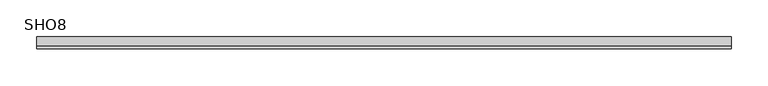
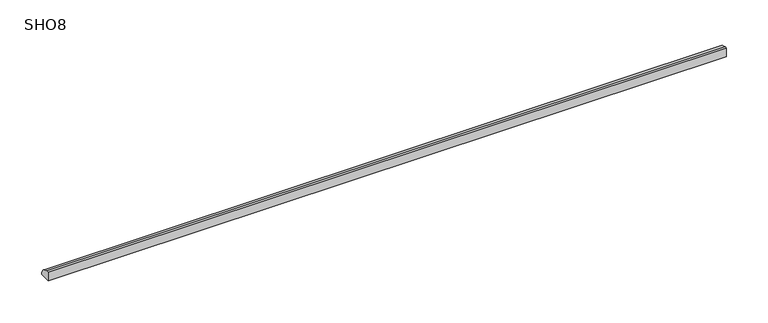
"""IFC4 building model written with IfcOpenShell, lengths in millimetres: proxy geometry, Molding-Merillat-Shoe : SHO8."""

from ifc_helpers import new_model, si_unit, point, frame, frame_2d, origin, place, context, project, spatial, polyline, circle_curve, trimmed, segment, composite_curve, outline, extrude, source, transform, mapped, element, save


def sho8_93cdf79d(model_context):
    return source(origin(), model_context, "Body", "SweptSolid", [
        extrude(outline(composite_curve([segment(polyline([(-15.875, 0.0), (-15.875, 12.7), (-12.7, 12.7)]), True, "CONTINUOUS"), segment(trimmed(circle_curve(frame_2d((-12.7, 0.0)), 12.7), [point((-12.7, 12.7))], [point((0.0, 0.0))], False, "CARTESIAN"), True, "CONTINUOUS"), segment(polyline([(0.0, 0.0), (-15.875, 0.0)]), True, "CONTINUOUS")], self_intersect=False)), frame((0.0, 0.0, 0.0), z_axis=(1.0, 0.0, 0.0), x_axis=(0.0, 1.0, 0.0)), (0.0, 0.0, 1.0), 939.8118988),
    ])


if __name__ == "__main__":
    model = new_model("IFC4")
    model_context = context("Model", 3, world=origin())
    ifc_project = project(units=[si_unit("LENGTHUNIT", "METRE", prefix="MILLI")], contexts=[model_context])
    site = spatial("IfcSite", under=ifc_project)
    building = spatial("IfcBuilding", under=site)
    placement = place(None, origin())
    sho8_shape = sho8_93cdf79d(model_context)
    element("IfcBuildingElementProxy", 1, Name="Molding-Merillat-Shoe : SHO8", ObjectType="Molding-Merillat-Shoe : SHO8", at=placement, inside=building, context=model_context, shape_type="MappedRepresentation", body=[
        mapped(sho8_shape, transform((0.0, 0.0, 0.0), x_axis=(1.0, 0.0, 0.0), y_axis=(0.0, 1.0, 0.0), z_axis=(0.0, 0.0, 1.0))),
    ])
    save(model, "model.ifc")

# Revit data of these elements
# Type "Molding-Merillat-Shoe : SHO8"
#   URL = "http://www.merillat.com/"
#   Product Page URL = "http://www.merillat.com/our-products/rooms/kitchen/"
#   Product Documentation Link = "http://merillatbusiness.com/wp-content/uploads/2014/07/Merillat_Classic_Catalog.pdf"
#   Model = "SHO8"
#   Manufacturer = "Merillat"
#   Description = "Molding"
#   Construction Notes = "Available in 8' Individual Sections or Cartons of 25 (SHO8-25)"
#   Assembly Code = "C3010130"
#   Width [instance default] = 1' - 0"
#   Height = 0' - 0 5/8"
#   Depth = 0' - 0 1/2"
#   Default Elevation = 4' - 0"
#   COBie.Type = no
#   Straight [instance default] = yes
#   Right Outside Corner [instance default] = no
#   Right Inside Corner [instance default] = no
#   Left Outside Corner [instance default] = no
#   Left Inside Corner [instance default] = no
#   Molding Material = Wood - Merillat - Hazelnut
#   Type Comments = ""
# Element 1 (IfcBuildingElementProxy, "Molding-Merillat-Shoe : SHO8")
#   Width = 3' - 1.00047"
#   Materials on its faces: "Wood - Merillat - Hazelnut"
# Materials
#   "Wood - Merillat - Hazelnut": class "Wood", colour RGB 138 103 81, transparency 0, Cost = 0
